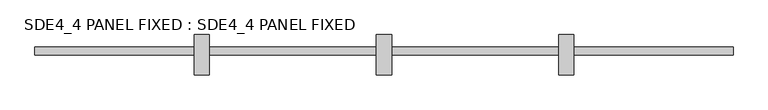
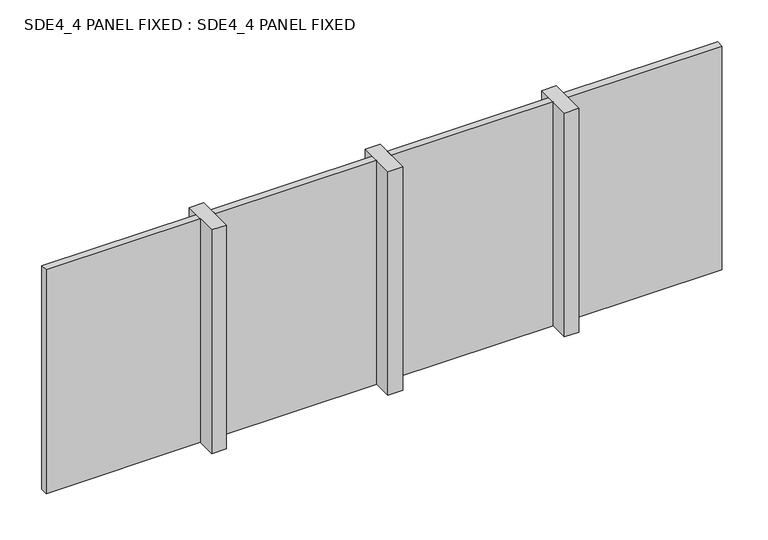
"""IFC4 building model written with IfcOpenShell, lengths in millimetres: plate geometry, SDE4_4 PANEL FIXED : SDE4_4 PANEL FIXED."""

from ifc_helpers import new_model, si_unit, origin, origin_with_axes, place, context, project, spatial, polyline, outline, extrude, source, transform, mapped, element, save


def sde4_4_panel_fixed_sde4_4_panel_fixed_71419ee0(model_context):
    return source(origin(), model_context, "Body", "SweptSolid", [
        extrude(outline(polyline([(-1150.0, 132.5), (-1150.0, -132.5), (-1250.0, -132.5), (-1250.0, 132.5), (-1150.0, 132.5)])), origin_with_axes(), (0.0, 0.0, 1.0), 1610.0),
        extrude(outline(polyline([(50.0, 132.5), (50.0, -132.5), (-50.0, -132.5), (-50.0, 132.5), (50.0, 132.5)])), origin_with_axes(), (0.0, 0.0, 1.0), 1610.0),
        extrude(outline(polyline([(1250.0, 132.5), (1250.0, -132.5), (1150.0, -132.5), (1150.0, 132.5), (1250.0, 132.5)])), origin_with_axes(), (0.0, 0.0, 1.0), 1610.0),
        extrude(outline(polyline([(2299.0, 50.0), (2299.0, 0.0), (1250.0, 0.0), (1250.0, 50.0), (2299.0, 50.0)])), origin_with_axes(), (0.0, 0.0, 1.0), 1610.0),
        extrude(outline(polyline([(1150.0, 50.0), (1150.0, 0.0), (50.0, 0.0), (50.0, 50.0), (1150.0, 50.0)])), origin_with_axes(), (0.0, 0.0, 1.0), 1610.0),
        extrude(outline(polyline([(-50.0, 50.0), (-50.0, 0.0), (-1150.0, 0.0), (-1150.0, 50.0), (-50.0, 50.0)])), origin_with_axes(), (0.0, 0.0, 1.0), 1610.0),
        extrude(outline(polyline([(-1250.0, 50.0), (-1250.0, 0.0), (-2300.0, 0.0), (-2300.0, 50.0), (-1250.0, 50.0)])), origin_with_axes(), (0.0, 0.0, 1.0), 1610.0),
    ])


if __name__ == "__main__":
    model = new_model("IFC4")
    model_context = context("Model", 3, world=origin())
    ifc_project = project(units=[si_unit("LENGTHUNIT", "METRE", prefix="MILLI")], contexts=[model_context])
    site = spatial("IfcSite", under=ifc_project)
    building = spatial("IfcBuilding", under=site)
    placement = place(None, origin())
    sde4_4_panel_fixed_sde4_4_panel_fixed_shape = sde4_4_panel_fixed_sde4_4_panel_fixed_71419ee0(model_context)
    element("IfcPlate", 1, ObjectType="SDE4_4 PANEL FIXED : SDE4_4 PANEL FIXED", at=placement, inside=building, context=model_context, shape_type="MappedRepresentation", body=[
        mapped(sde4_4_panel_fixed_sde4_4_panel_fixed_shape, transform((0.0, 0.0, 0.0), x_axis=(1.0, 0.0, 0.0), y_axis=(0.0, 1.0, 0.0), z_axis=(0.0, 0.0, 1.0))),
    ])
    save(model, "model.ifc")

# Revit data of these elements
# Type "SDE4_4 PANEL FIXED : SDE4_4 PANEL FIXED"
#   Type Mark = "CW-GLASS"
#   Analytic Construction = "<None>"
#   Glass = Glass
#   Frame = Aluminium
# Element 1 (IfcPlate, "SDE4_4 PANEL FIXED : SDE4_4 PANEL FIXED")
#   Materials on its faces: "Glass", "Aluminium"
# Materials
#   "Glass": class "Glass", colour RGB 0 128 192, transparency 0.9, Keynote = "L40", Cost = 0
#   "Aluminium": class "Unassigned", colour RGB 247 247 247, transparency 0, Cost = 0
